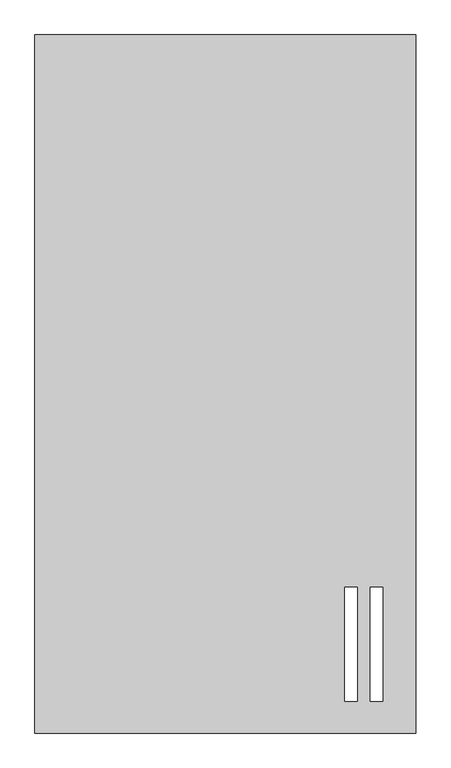
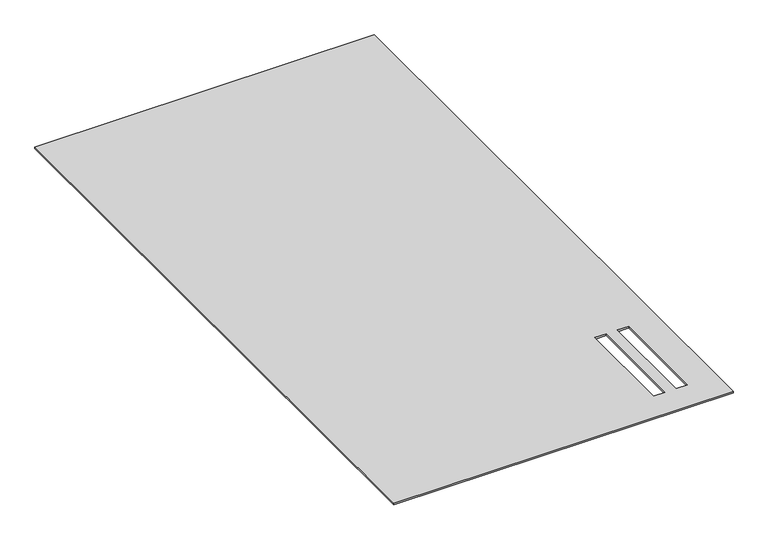
"""IFC4 building model written with IfcOpenShell, lengths in millimetres: proxy geometry, TSP Geyser Solar 200L : TSP Geyser Solar 200L."""

from ifc_helpers import new_model, si_unit, origin, origin_with_axes, place, context, project, spatial, polyline, outline, extrude, source, transform, mapped, element, save


def electrical_fixtures_7282ffa6(model_context):
    return source(origin(), model_context, "Body", "SweptSolid", [
        extrude(outline(polyline([(-600.0, 600.0), (0.0, 600.0), (0.0, -500.0), (-600.0, -500.0), (-600.0, 600.0)]), holes=[polyline([(-71.8082825, -450.0), (-51.8082825, -450.0), (-51.8082825, -270.0), (-71.8082825, -270.0), (-71.8082825, -450.0)]), polyline([(-111.8082825, -450.0), (-91.8082825, -450.0), (-91.8082825, -270.0), (-111.8082825, -270.0), (-111.8082825, -450.0)])]), origin_with_axes(), (0.0, 0.0, 1.0), 3.0),
    ])


if __name__ == "__main__":
    model = new_model("IFC4")
    model_context = context("Model", 3, world=origin())
    ifc_project = project(units=[si_unit("LENGTHUNIT", "METRE", prefix="MILLI")], contexts=[model_context])
    site = spatial("IfcSite", under=ifc_project)
    building = spatial("IfcBuilding", under=site)
    placement = place(None, origin())
    electrical_fixtures_shape = electrical_fixtures_7282ffa6(model_context)
    element("IfcBuildingElementProxy", 1, Name="TSP Geyser Solar 200L : TSP Geyser Solar 200L", ObjectType="TSP Geyser Solar 200L : TSP Geyser Solar 200L", at=placement, inside=building, context=model_context, shape_type="MappedRepresentation", body=[
        mapped(electrical_fixtures_shape, transform((0.0, 0.0, 0.0), x_axis=(1.0, 0.0, 0.0), y_axis=(0.0, 1.0, 0.0), z_axis=(0.0, 0.0, 1.0))),
    ])
    save(model, "model.ifc")

# Revit data of these elements
# Type "TSP Geyser Solar 200L : TSP Geyser Solar 200L"
#   Model = "TSP_SGEY200"
#   Default Elevation = 0
# Element 1 (IfcBuildingElementProxy, "TSP Geyser Solar 200L : TSP Geyser Solar 200L")
#   Materials on its faces: "Aluminum, Anodized Red"
# Materials
#   "Aluminum, Anodized Red": class "Metal", colour RGB 120 120 120, transparency 0, Description = "Anodized aluminum, red", Cost = 0
